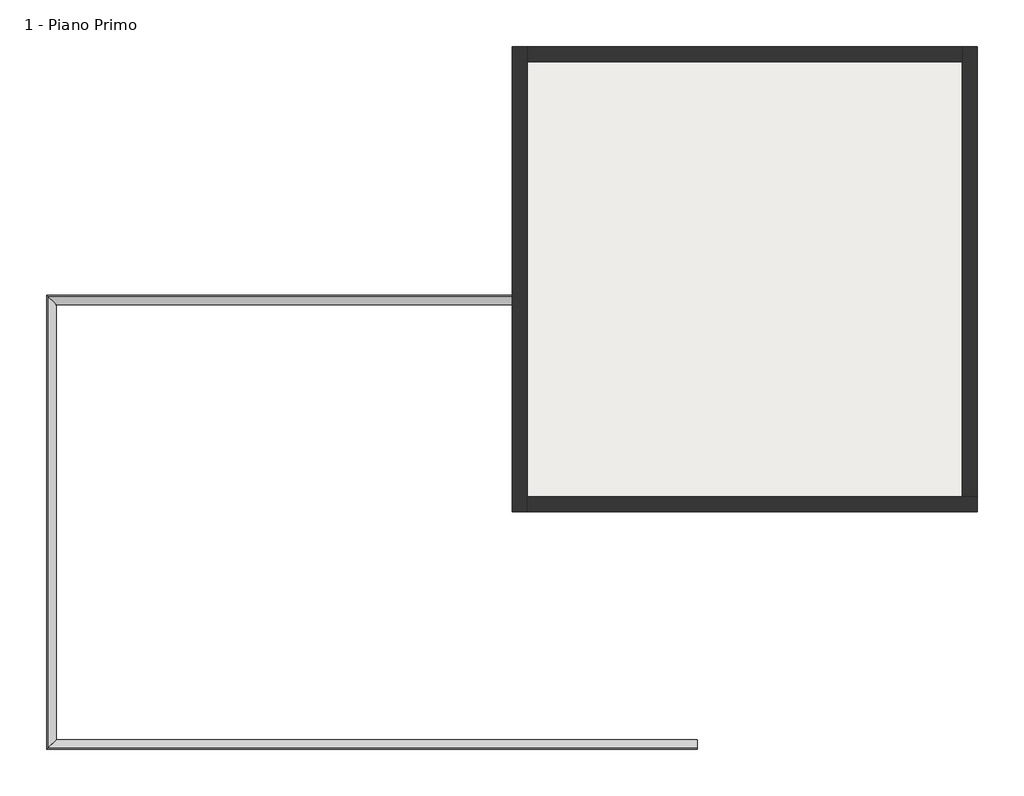
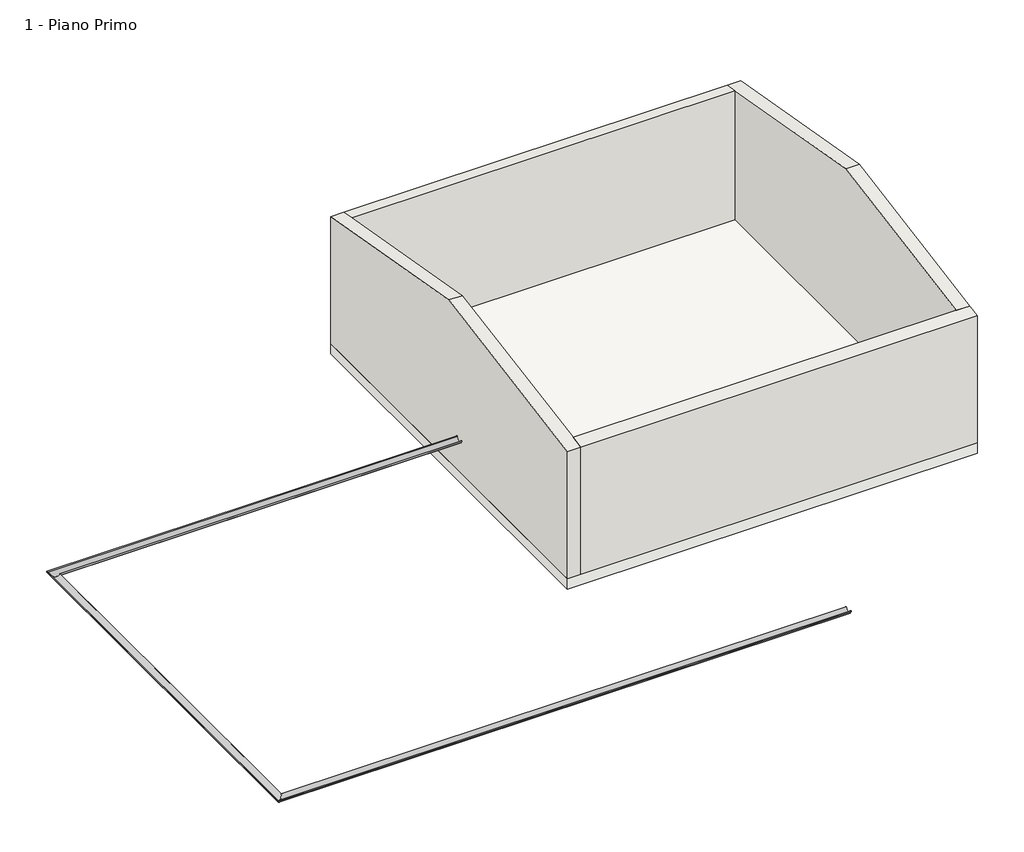
# One storey: 4 walls, 1 pipe segment, 1 slab.
"""IFC4 building model written with IfcOpenShell, lengths in millimetres."""

import ifcopenshell
import ifcopenshell.guid

model = None  # the IFC model being written
_history = None  # IfcOwnerHistory: only IFC2X3 demands one
_inside = {}  # id of a spatial element -> (the spatial element, [elements in it])
_under = {}  # id of a project, library or spatial element -> (it, [spatial elements below it])
_declared = {}  # id of a project -> (the project, [libraries it declares])
_typed = {}  # id of a type object -> (the type object, [elements of that type])
_made_of = {}  # id of a material, layer set ... -> (it, [elements and type objects made of it])


def new_model(schema):
    """Start an empty IFC model of exactly this schema.

    Asked for "IFC4X3", IfcOpenShell would pick the latest addendum, in which some entities
    have other attributes; the version numbers below select the first issue.
    IFC2X3 requires an IfcOwnerHistory on every rooted entity: one is made here for all.
    """
    global model, _history
    if schema == "IFC4X3":
        model = ifcopenshell.file(schema_version=(4, 3, 0, 0))
    else:
        model = ifcopenshell.file(schema=schema)
    _inside.clear()
    _under.clear()
    _declared.clear()
    _typed.clear()
    _made_of.clear()
    _history = None
    if model.schema == "IFC2X3":
        org = make("IfcOrganization", Name="unknown")
        user = make(
            "IfcPersonAndOrganization",
            ThePerson=make("IfcPerson", FamilyName="unknown"),
            TheOrganization=org,
        )
        app = make(
            "IfcApplication",
            ApplicationDeveloper=org,
            Version="unknown",
            ApplicationFullName="unknown",
            ApplicationIdentifier="unknown",
        )
        _history = make(
            "IfcOwnerHistory",
            OwningUser=user,
            OwningApplication=app,
            ChangeAction="ADDED",
            CreationDate=0,
        )
    return model


def make(cls, **values):
    """One entity of the class cls with the attributes given. An attribute that is None is left unset."""
    return model.create_entity(
        cls, **{name: value for name, value in values.items() if value is not None}
    )


def rooted(cls, **values):
    """An entity with a GlobalId (a new one), such as an element, a storey or a relation."""
    return make(cls, GlobalId=ifcopenshell.guid.new(), OwnerHistory=_history, **values)


def si_unit(unit_type, name, prefix=None):
    """IfcSIUnit, for example si_unit("LENGTHUNIT", "METRE", prefix="MILLI")."""
    return make("IfcSIUnit", UnitType=unit_type, Prefix=prefix, Name=name)


def assignment(units):
    """IfcUnitAssignment: the units of a project."""
    return None if units is None else make("IfcUnitAssignment", Units=units)


def point(xyz):
    """IfcCartesianPoint."""
    return None if xyz is None else make("IfcCartesianPoint", Coordinates=xyz)


def direction(xyz):
    """IfcDirection."""
    return None if xyz is None else make("IfcDirection", DirectionRatios=xyz)


def frame(location, z_axis=None, x_axis=None):
    """IfcAxis2Placement3D, a coordinate frame: its origin and axes. An axis left out is left unset."""
    return make(
        "IfcAxis2Placement3D",
        Location=point(location),
        Axis=direction(z_axis),
        RefDirection=direction(x_axis),
    )


def origin():
    """The frame at (0, 0, 0) with its axes left unset."""
    return frame((0.0, 0.0, 0.0))


def place(relative_to, where):
    """IfcLocalPlacement: puts the frame where relative to a parent placement (None: the world)."""
    return make(
        "IfcLocalPlacement", PlacementRelTo=relative_to, RelativePlacement=where
    )


def context(
    kind, dimensions, precision=None, world=None, true_north=None, identifier=None
):
    """IfcGeometricRepresentationContext, for example the 3D "Model" context."""
    return make(
        "IfcGeometricRepresentationContext",
        ContextIdentifier=identifier,
        ContextType=kind,
        CoordinateSpaceDimension=dimensions,
        Precision=precision,
        WorldCoordinateSystem=world,
        TrueNorth=true_north,
    )


def project(units=None, contexts=None):
    """IfcProject with its units and contexts."""
    return rooted(
        "IfcProject",
        Name="project",
        RepresentationContexts=contexts,
        UnitsInContext=assignment(units),
    )


def spatial(cls, under=None, at=None, **own):
    """A site, building, storey or space (cls), placed at a placement, below another one or the project."""
    s = rooted(cls, ObjectPlacement=at, **own)
    if under is not None:
        _under.setdefault(under.id(), (under, []))[1].append(s)
    return s


def polyline(points):
    """IfcPolyline through the points."""
    return make("IfcPolyline", Points=[point(p) for p in points])


def circle_curve(where, radius):
    """IfcCircle in the frame where."""
    return make("IfcCircle", Position=where, Radius=radius)


def ellipse_curve(where, semi_axis1, semi_axis2):
    """IfcEllipse in the frame where."""
    return make(
        "IfcEllipse", Position=where, SemiAxis1=semi_axis1, SemiAxis2=semi_axis2
    )


def outline(outer, holes=None, kind="AREA"):
    """IfcArbitraryClosedProfileDef: a profile drawn as a closed curve; with holes, ...WithVoids."""
    if holes is None:
        return make("IfcArbitraryClosedProfileDef", ProfileType=kind, OuterCurve=outer)
    return make(
        "IfcArbitraryProfileDefWithVoids",
        ProfileType=kind,
        OuterCurve=outer,
        InnerCurves=holes,
    )


def extrude(swept, where, along, depth):
    """IfcExtrudedAreaSolid: the profile swept, set in the frame where, extruded along a direction by depth."""
    return make(
        "IfcExtrudedAreaSolid",
        SweptArea=swept,
        Position=where,
        ExtrudedDirection=direction(along),
        Depth=depth,
    )


def faces_of(points, faces, orient=None, outer=None):
    """IfcFace entities. A face is a list of loops; a loop is a list of indices into points, from 0.

    orient and outer hold one flag for each loop. By default every Orientation is true, the
    first loop of a face is its IfcFaceOuterBound and the others are IfcFaceBound.
    """
    made = []
    for i, loops in enumerate(faces):
        bounds = []
        for j, loop in enumerate(loops):
            is_outer = j == 0 if outer is None else outer[i][j]
            bounds.append(
                make(
                    "IfcFaceOuterBound" if is_outer else "IfcFaceBound",
                    Bound=make("IfcPolyLoop", Polygon=[points[k] for k in loop]),
                    Orientation=True if orient is None else orient[i][j],
                )
            )
        made.append(make("IfcFace", Bounds=bounds))
    return made


def faceted_brep(points, faces, orient=None, outer=None, voids=None):
    """IfcFacetedBrep: a solid bounded by flat faces; with voids (closed shells), ...WithVoids."""
    shared = [point(p) for p in points]
    hull = make("IfcClosedShell", CfsFaces=faces_of(shared, faces, orient, outer))
    if voids is None:
        return make("IfcFacetedBrep", Outer=hull)
    return make(
        "IfcFacetedBrepWithVoids",
        Outer=hull,
        Voids=[
            make(cls, CfsFaces=faces_of(shared, fs, o, b)) for cls, fs, o, b in voids
        ],
    )


def shape(context_of_items, identifier, shape_type, items):
    """IfcShapeRepresentation: the items that make up one representation, for example the "Body"."""
    return make(
        "IfcShapeRepresentation",
        ContextOfItems=context_of_items,
        RepresentationIdentifier=identifier,
        RepresentationType=shape_type,
        Items=items,
    )


def made_of(thing, what):
    """Note that an element or type object is made of a material, layer set ...; save() writes the relation."""
    if what is not None:
        _made_of.setdefault(what.id(), (what, []))[1].append(thing)
    return thing


def element(
    cls,
    number,
    at=None,
    inside=None,
    cuts=None,
    type_object=None,
    material=None,
    context=None,
    identifier="Body",
    shape_type=None,
    held_by="IfcProductDefinitionShape",
    body=None,
    shapes=None,
    **own,
):
    """One element of the class cls, such as IfcWall. Its Tag is "e" and its number.

    at: its placement. inside: the storey or other place that contains it. cuts: it is an
    opening in that element (IfcRelVoidsElement). A single representation is given by context,
    identifier, shape_type and body (its items); several are given by shapes. held_by: the class
    of the entity that holds the representations. save() writes the other relations.
    """
    e = rooted(cls, Tag="e%d" % number, ObjectPlacement=at, **own)
    if body is not None:
        shapes = [shape(context, identifier, shape_type, body)]
    if shapes is not None:
        e.Representation = make(held_by, Representations=shapes)
    if inside is not None:
        _inside.setdefault(inside.id(), (inside, []))[1].append(e)
    if cuts is not None:
        rooted(
            "IfcRelVoidsElement", RelatingBuildingElement=cuts, RelatedOpeningElement=e
        )
    if type_object is not None:
        _typed.setdefault(type_object.id(), (type_object, []))[1].append(e)
    return made_of(e, material)


def aggregate(whole, parts):
    """IfcRelAggregates: a whole, such as a stair, and the parts it consists of."""
    return rooted("IfcRelAggregates", RelatingObject=whole, RelatedObjects=parts)


def save(model, path):
    """Write the relations noted so far, then the file.

    IfcRelAggregates (storeys below a building ...), IfcRelContainedInSpatialStructure (elements
    in a storey), IfcRelDefinesByType, IfcRelAssociatesMaterial and IfcRelDeclares: one each for
    every whole, place, type object, material and project.
    """
    for whole, parts in _under.values():
        aggregate(whole, parts)
    for where, things in _inside.values():
        rooted(
            "IfcRelContainedInSpatialStructure",
            RelatedElements=things,
            RelatingStructure=where,
        )
    for kind, things in _typed.values():
        rooted("IfcRelDefinesByType", RelatedObjects=things, RelatingType=kind)
    for what, things in _made_of.values():
        rooted("IfcRelAssociatesMaterial", RelatedObjects=things, RelatingMaterial=what)
    for by, libraries in _declared.values():
        rooted("IfcRelDeclares", RelatingContext=by, RelatedDefinitions=libraries)
    model.write(path)


def plane_surface(at):
    """IfcPlane: the flat surface through the origin of the frame at, square to its z axis."""
    return make("IfcPlane", Position=at)


def cylinder_surface(at, radius):
    """IfcCylindricalSurface: all points at the distance radius from the z axis of the frame at."""
    return make("IfcCylindricalSurface", Position=at, Radius=radius)


def revolved_surface(curve, axis_point, axis_direction):
    """IfcSurfaceOfRevolution: the curve turned about the line through axis_point along axis_direction."""
    return make(
        "IfcSurfaceOfRevolution",
        SweptCurve=make("IfcArbitraryOpenProfileDef", ProfileType="CURVE", Curve=curve),
        AxisPosition=make("IfcAxis1Placement", Location=point(axis_point), Axis=direction(axis_direction)),
    )


def advanced_brep(points, edges, surfaces, faces):
    """IfcAdvancedBrep: a solid bounded by faces that lie on surfaces and meet in shared edges.

    An edge is (start, end): straight between two places in points (the first is 0);
    or (start, end, curve); or (start, end, curve, False) where it runs against its curve.
    A face is (place in surfaces, loops), or (place, loops, False) where it looks against
    its surface's normal. A loop lists edges by number (the first is 1), with a minus sign
    where the edge is run from its end to its start. The first loop is the outer one.
    """
    corners = [point(p) for p in points]
    vertices = [make("IfcVertexPoint", VertexGeometry=c) for c in corners]
    made = []
    for start, end, *more in edges:
        made.append(
            make(
                "IfcEdgeCurve",
                EdgeStart=vertices[start],
                EdgeEnd=vertices[end],
                EdgeGeometry=more[0] if more else make("IfcPolyline", Points=[corners[start], corners[end]]),
                SameSense=more[1] if len(more) > 1 else True,
            )
        )
    hull = []
    for where, loops, *sense in faces:
        bounds = []
        for j, loop in enumerate(loops):
            ring = [make("IfcOrientedEdge", EdgeElement=made[abs(k) - 1], Orientation=k > 0) for k in loop]
            bounds.append(
                make(
                    "IfcFaceOuterBound" if j == 0 else "IfcFaceBound",
                    Bound=make("IfcEdgeLoop", EdgeList=ring),
                    Orientation=True,
                )
            )
        hull.append(make("IfcAdvancedFace", Bounds=bounds, FaceSurface=surfaces[where], SameSense=sense[0] if sense else True))
    return make("IfcAdvancedBrep", Outer=make("IfcClosedShell", CfsFaces=hull))


model = new_model("IFC4")

# Units and contexts
model_context = context("Model", 3, world=origin())
ifc_project = project(units=[si_unit("LENGTHUNIT", "METRE", prefix="MILLI")], contexts=[model_context])

# Site, building, storey
site = spatial("IfcSite", under=ifc_project)
building = spatial("IfcBuilding", under=site)
storey = spatial("IfcBuildingStorey", under=building, Name="1 - Piano Primo", Elevation=4000.0)

# Pipe segment
placement = place(None, origin())
element("IfcPipeSegment", 1, ObjectType="Grondaia", at=placement, inside=storey, context=model_context, shape_type="AdvancedBrep", body=[
    advanced_brep(
    [(-1450.292668, 3378.2301644, 4973.2050808), (-1450.292668, 3588.4212472, 4973.2050808), (-1450.292668, 3586.4212472, 4973.2050808), (-1450.292668, 3380.2301644, 4973.2050808), (-1450.292668, 3368.2301644, 4961.2050808), (-1450.292668, 3368.2301644, 4963.2050808), (-17240.4837508, 3368.2301644, 4963.2050808), (-17230.4837508, 3378.2301644, 4973.2050808), (-17240.4837508, 3368.2301644, 4961.2050808), (-17228.4837508, 3380.2301644, 4973.2050808), (-17022.292668, 3586.4212472, 4973.2050808), (-17020.292668, 3588.4212472, 4973.2050808), (-17240.4837508, 14378.61233, 4963.2050808), (-17230.4837508, 14368.61233, 4973.2050808), (-17240.4837508, 14378.61233, 4961.2050808), (-17228.4837508, 14366.61233, 4973.2050808), (-17022.292668, 14160.4212472, 4973.2050808), (-17020.292668, 14158.4212472, 4973.2050808), (-5941.300812, 14368.61233, 4973.2050808), (-5941.300812, 14378.61233, 4963.2050808), (-5941.300812, 14378.61233, 4961.2050808), (-5941.300812, 14366.61233, 4973.2050808), (-5941.300812, 14160.4212472, 4973.2050808), (-5941.300812, 14158.4212472, 4973.2050808)],
    [
        (0, 1, circle_curve(frame((-1450.292668, 3483.3257058, 4973.2050808), z_axis=(1.0, 0.0, 0.0), x_axis=(0.0, -1.0, 0.0)), 105.0955414)),
        (1, 2),
        (2, 3, circle_curve(frame((-1450.292668, 3483.3257058, 4973.2050808), z_axis=(-1.0, 0.0, 0.0), x_axis=(0.0, -1.0, 0.0)), 103.0955414)),
        (3, 4, circle_curve(frame((-1450.292668, 3368.2301644, 4973.2050808), z_axis=(1.0, 0.0, 0.0), x_axis=(0.0, -1.0, 0.0)), 12.0)),
        (4, 5),
        (5, 0, circle_curve(frame((-1450.292668, 3368.2301644, 4973.2050808), z_axis=(-1.0, 0.0, 0.0), x_axis=(0.0, -1.0, 0.0)), 10.0)),
        (6, 7, ellipse_curve(frame((-17240.4837508, 3368.2301644, 4973.2050808), z_axis=(-0.7071067811865469, 0.7071067811865481, 0.0), x_axis=(0.7071067811865481, 0.7071067811865468, 0.0)), 14.1421356, 10.0)),
        (7, 0),
        (5, 6),
        (8, 6),
        (4, 8),
        (9, 8, ellipse_curve(frame((-17240.4837508, 3368.2301644, 4973.2050808), z_axis=(0.7071067811865469, -0.7071067811865481, 0.0), x_axis=(-0.7071067811865481, -0.7071067811865468, 0.0)), 16.9705627, 12.0)),
        (3, 9),
        (10, 9, ellipse_curve(frame((-17125.3882094, 3483.3257058, 4973.2050808), z_axis=(-0.7071067811865469, 0.7071067811865481, 0.0), x_axis=(0.7071067811865481, 0.7071067811865468, 0.0)), 145.7991129, 103.0955414)),
        (2, 10),
        (11, 10),
        (1, 11),
        (7, 11, ellipse_curve(frame((-17125.3882094, 3483.3257058, 4973.2050808), z_axis=(0.7071067811865469, -0.7071067811865481, 0.0), x_axis=(-0.7071067811865481, -0.7071067811865468, 0.0)), 148.62754, 105.0955414)),
        (12, 13, ellipse_curve(frame((-17240.4837508, 14378.61233, 4973.2050808), z_axis=(0.7071067811865491, 0.7071067811865458, 0.0), x_axis=(0.7071067811865456, -0.7071067811865493, 0.0)), 14.1421356, 10.0)),
        (13, 7),
        (6, 12),
        (14, 12),
        (8, 14),
        (15, 14, ellipse_curve(frame((-17240.4837508, 14378.61233, 4973.2050808), z_axis=(-0.7071067811865491, -0.7071067811865458, 0.0), x_axis=(-0.7071067811865456, 0.7071067811865493, 0.0)), 16.9705627, 12.0)),
        (9, 15),
        (16, 15, ellipse_curve(frame((-17125.3882094, 14263.5167886, 4973.2050808), z_axis=(0.7071067811865491, 0.7071067811865458, 0.0), x_axis=(0.7071067811865456, -0.7071067811865493, 0.0)), 145.7991129, 103.0955414)),
        (10, 16),
        (17, 16),
        (11, 17),
        (13, 17, ellipse_curve(frame((-17125.3882094, 14263.5167886, 4973.2050808), z_axis=(-0.7071067811865491, -0.7071067811865458, 0.0), x_axis=(-0.7071067811865456, 0.7071067811865493, 0.0)), 148.62754, 105.0955414)),
        (18, 19, circle_curve(frame((-5941.300812, 14378.61233, 4973.2050808), z_axis=(-1.0, 0.0, 0.0), x_axis=(0.0, 1.0, 0.0)), 10.0)),
        (19, 20),
        (20, 21, circle_curve(frame((-5941.300812, 14378.61233, 4973.2050808), z_axis=(1.0, 0.0, 0.0), x_axis=(0.0, 1.0, 0.0)), 12.0)),
        (21, 22, circle_curve(frame((-5941.300812, 14263.5167886, 4973.2050808), z_axis=(-1.0, 0.0, 0.0), x_axis=(0.0, 1.0, 0.0)), 103.0955414)),
        (22, 23),
        (23, 18, circle_curve(frame((-5941.300812, 14263.5167886, 4973.2050808), z_axis=(1.0, 0.0, 0.0), x_axis=(0.0, 1.0, 0.0)), 105.0955414)),
        (18, 13),
        (12, 19),
        (14, 20),
        (15, 21),
        (16, 22),
        (17, 23),
    ],
    [
        plane_surface(frame((-1450.292668, 3588.4212472, 4741.5716357), z_axis=(1.0, 0.0, 0.0), x_axis=(0.0, 1.0, 0.0))),
        revolved_surface(polyline([(-1450.292668, 3358.2301644, 4973.2050808), (-17250.483750783216, 3358.2301644, 4973.2050808)]), (-17020.292668, 3368.2301644, 4973.2050808), (1.0, 0.0, 0.0)),
        plane_surface(frame((-17240.4837508, 3368.2301644, 4963.2050808), z_axis=(0.0, 1.0, 0.0), x_axis=(1.0, 0.0, 0.0))),
        cylinder_surface(frame((-17020.292668, 3368.2301644, 4973.2050808), z_axis=(-1.0, 0.0, 0.0), x_axis=(0.0, -1.0, 0.0)), 12.0),
        revolved_surface(polyline([(-1450.292668, 3380.2301644, 4973.2050808), (-17228.483750822572, 3380.2301644, 4973.2050808)]), (-17020.292668, 3483.3257058, 4973.2050808), (1.0, 0.0, 0.0)),
        plane_surface(frame((-17022.292668, 3586.4212472, 4973.2050808), z_axis=(0.0, 0.0, 1.0), x_axis=(1.0, 0.0, 0.0))),
        cylinder_surface(frame((-17020.292668, 3483.3257058, 4973.2050808), z_axis=(-1.0, 0.0, 0.0), x_axis=(0.0, -1.0, 0.0)), 105.0955414),
        revolved_surface(polyline([(-17250.4837508, 3358.23016441678, 4973.2050808), (-17250.4837508, 14388.61232998322, 4973.2050808)]), (-17240.4837508, 14158.4212472, 4973.2050808), (0.0, -1.0, 0.0)),
        plane_surface(frame((-17240.4837508, 14378.61233, 4963.2050808), z_axis=(1.0, 0.0, 0.0), x_axis=(0.0, -1.0, 0.0))),
        cylinder_surface(frame((-17240.4837508, 14158.4212472, 4973.2050808), z_axis=(0.0, 1.0, 0.0), x_axis=(-1.0, 0.0, 0.0)), 12.0),
        revolved_surface(polyline([(-17228.4837508, 3380.2301643774263, 4973.2050808), (-17228.4837508, 14366.612330022574, 4973.2050808)]), (-17125.3882094, 14158.4212472, 4973.2050808), (0.0, -1.0, 0.0)),
        plane_surface(frame((-17022.292668, 14160.4212472, 4973.2050808), z_axis=(0.0, 0.0, 1.0), x_axis=(0.0, -1.0, 0.0))),
        cylinder_surface(frame((-17125.3882094, 14158.4212472, 4973.2050808), z_axis=(0.0, 1.0, 0.0), x_axis=(-1.0, 0.0, 0.0)), 105.0955414),
        plane_surface(frame((-5941.300812, 14158.4212472, 4741.5716357), z_axis=(1.0, 0.0, 0.0), x_axis=(0.0, -1.0, 0.0))),
        revolved_surface(polyline([(-17250.483750783216, 14388.61233, 4973.2050808), (-5941.300812, 14388.61233, 4973.2050808)]), (-5941.300812, 14378.61233, 4973.2050808), (-1.0, 0.0, 0.0)),
        plane_surface(frame((-5941.300812, 14378.61233, 4963.2050808), z_axis=(0.0, -1.0, 0.0), x_axis=(-1.0, 0.0, 0.0))),
        cylinder_surface(frame((-5941.300812, 14378.61233, 4973.2050808), z_axis=(1.0, 0.0, 0.0), x_axis=(0.0, 1.0, 0.0)), 12.0),
        revolved_surface(polyline([(-17228.483750822572, 14366.61233, 4973.2050808), (-5941.300812, 14366.61233, 4973.2050808)]), (-5941.300812, 14263.5167886, 4973.2050808), (-1.0, 0.0, 0.0)),
        plane_surface(frame((-5941.300812, 14160.4212472, 4973.2050808), z_axis=(0.0, 0.0, 1.0), x_axis=(-1.0, 0.0, 0.0))),
        cylinder_surface(frame((-5941.300812, 14263.5167886, 4973.2050808), z_axis=(1.0, 0.0, 0.0), x_axis=(0.0, 1.0, 0.0)), 105.0955414),
    ],
    [
        (0, [[1, 2, 3, 4, 5, 6]]),
        (1, [[7, 8, -6, 9]]),
        (2, [[10, -9, -5, 11]]),
        (3, [[12, -11, -4, 13]]),
        (4, [[14, -13, -3, 15]]),
        (5, [[16, -15, -2, 17]]),
        (6, [[18, -17, -1, -8]]),
        (7, [[19, 20, -7, 21]]),
        (8, [[22, -21, -10, 23]]),
        (9, [[24, -23, -12, 25]]),
        (10, [[26, -25, -14, 27]]),
        (11, [[28, -27, -16, 29]]),
        (12, [[30, -29, -18, -20]]),
        (13, [[31, 32, 33, 34, 35, 36]]),
        (14, [[-31, 37, -19, 38]]),
        (15, [[-32, -38, -22, 39]]),
        (16, [[-33, -39, -24, 40]]),
        (17, [[-34, -40, -26, 41]]),
        (18, [[-35, -41, -28, 42]]),
        (19, [[-36, -42, -30, -37]]),
    ],
),
])

# Slab
element("IfcSlab", 2, ObjectType="Latero Cementizio - 30 cm", at=placement, inside=storey, context=model_context, shape_type="SweptSolid", body=[
    extrude(outline(polyline([(-5941.300812, 20428.4386987), (5358.699188, 20428.4386987), (5358.699188, 9128.4386987), (-5941.300812, 9128.4386987), (-5941.300812, 20428.4386987)])), frame((0.0, 0.0, 3700.0), z_axis=(0.0, 0.0, 1.0), x_axis=(1.0, 0.0, 0.0)), (0.0, 0.0, 1.0), 300.0),
])

# Walls
element("IfcWall", 3, ObjectType="37 cm", at=placement, inside=storey, context=model_context, shape_type="Brep", body=[
    faceted_brep([(-5941.300812, 20428.4386987, 4000.0), (-5941.300812, 9128.4386987, 4000.0), (-5941.300812, 9128.4386987, 7700.0), (-5941.300812, 14778.4386987, 8696.247441), (-5941.300812, 20428.4386987, 7700.0), (-5571.300812, 20428.4386987, 4000.0), (-5571.300812, 20428.4386987, 7700.0), (-5571.300812, 20058.4386987, 7765.2409829), (-5571.300812, 14778.4386987, 8696.247441), (-5571.300812, 9498.4386987, 7765.2409829), (-5571.300812, 9128.4386987, 7700.0), (-5571.300812, 9128.4386987, 4000.0), (-5571.300812, 9498.4386987, 4000.0), (-5571.300812, 20058.4386987, 4000.0)], [[[0, 1, 2, 3, 4]], [[5, 6, 7, 8, 9, 10, 11, 12, 13]], [[1, 0, 5, 13, 12, 11]], [[2, 1, 11, 10]], [[0, 4, 6, 5]], [[4, 3, 8, 7, 6]], [[3, 2, 10, 9, 8]]]),
])
element("IfcWall", 4, ObjectType="37 cm", at=placement, inside=storey, context=model_context, shape_type="Brep", body=[
    faceted_brep([(-5571.300812, 9128.4386987, 4000.0), (5358.699188, 9128.4386987, 4000.0), (5358.699188, 9128.4386987, 7700.0), (-5571.300812, 9128.4386987, 7700.0), (-5571.300812, 9498.4386987, 4000.0), (-5571.300812, 9498.4386987, 7765.2409829), (4988.699188, 9498.4386987, 7765.2409829), (5358.699188, 9498.4386987, 7765.2409829), (5358.699188, 9498.4386987, 4000.0), (4988.699188, 9498.4386987, 4000.0)], [[[0, 1, 2, 3]], [[4, 5, 6, 7, 8, 9]], [[1, 0, 4, 9, 8]], [[0, 3, 5, 4]], [[2, 1, 8, 7]], [[3, 2, 7, 6, 5]]]),
])
element("IfcWall", 5, ObjectType="37 cm", at=placement, inside=storey, context=model_context, shape_type="Brep", body=[
    faceted_brep([(5358.699188, 9498.4386987, 4000.0), (5358.699188, 20428.4386987, 4000.0), (5358.699188, 20428.4386987, 7700.0), (5358.699188, 14778.4386987, 8696.247441), (5358.699188, 9498.4386987, 7765.2409829), (4988.699188, 9498.4386987, 4000.0), (4988.699188, 9498.4386987, 7765.2409829), (4988.699188, 14778.4386987, 8696.247441), (4988.699188, 20058.4386987, 7765.2409829), (4988.699188, 20428.4386987, 7700.0), (4988.699188, 20428.4386987, 4000.0), (4988.699188, 20058.4386987, 4000.0)], [[[0, 1, 2, 3, 4]], [[5, 6, 7, 8, 9, 10, 11]], [[1, 0, 5, 11, 10]], [[0, 4, 6, 5]], [[2, 1, 10, 9]], [[4, 3, 7, 6]], [[3, 2, 9, 8, 7]]]),
])
element("IfcWall", 6, ObjectType="37 cm", at=placement, inside=storey, context=model_context, shape_type="SweptSolid", body=[
    extrude(outline(polyline([(20428.4386987, 7700.0), (20428.4386987, 4000.0), (20058.4386987, 4000.0), (20058.4386987, 7765.2409829), (20428.4386987, 7700.0)])), frame((-5571.300812, 0.0, 0.0), z_axis=(1.0, 0.0, 0.0), x_axis=(0.0, 1.0, 0.0)), (0.0, 0.0, 1.0), 10560.0),
])

save(model, "model.ifc")

# Revit data of these elements
# Type "Latero Cementizio - 30 cm"
#   Keynote = "S/3"
#   Function = 0
#   Layers, outside or top first: 0.02 m "Ceramica bianca" (function 4); 0.065 m "Sabbia e Calcestruzzo" (function 2); 0.04 m "Calcestruzzo" (function 1); 0.16 m "Laterizio (2)" (function 1); 0.015 m "Intonaco - Bianco" (function 5)
# Type "37 cm"
#   Keynote = "Mb/3"
#   Layers, outside or top first: 0.02 m "Intonaco esterno" (function 1); 0.08 m "Isolamento" (function 1); 0.25 m "Calcestruzzo Blocchi" (function 1); 0.02 m "Intonaco interno" (function 5)
# Element 1 (IfcPipeSegment, "Grondaia")
#   Phase Created = Stato di Progetto
#   Materials on its faces: "Default - Grondaia"
# Element 2 (IfcSlab, "Latero Cementizio - 30 cm")
#   Height Offset From Level = 0.00 m
#   Phase Created = Stato di Progetto
#   Materials on its faces: "Intonaco - Bianco", "Ceramica bianca"
# Element 3 (IfcWall, "37 cm")
#   Top Offset = 0.00 m
#   Base Offset = 0.00 m
#   Unconnected Height = 3.70 m
#   wall height = 3.70 m
#   Phase Created = Stato di Progetto
#   Base Constraint = 1 - Piano Primo
#   Materials on its faces: "Intonaco interno", "Default - Calcestruzzo", "Intonaco esterno"
# Elements 4, 5, 6 (IfcWall, "37 cm")
#   Top Offset = 0.00 m
#   Base Offset = 0.00 m
#   Unconnected Height = 3.70 m
#   wall height = 3.70 m
#   Phase Created = Stato di Progetto
#   Base Constraint = 1 - Piano Primo
#   Materials on its faces: "Default - Calcestruzzo", "Intonaco interno", "Intonaco esterno"
# Materials
#   "Ceramica bianca": class "Ceramica", colour RGB 210 210 210, transparency 0, Description = "Finitura interna - Piastrelle di ceramica incollate", Cost = 0
#   "Sabbia e Calcestruzzo": class "Calcestruzzo", colour RGB 127 127 127, transparency 0, Description = "Magrone - Sabbia e cemento", Cost = 0
#   "Calcestruzzo": class "Calcestruzzo", colour RGB 192 192 192, transparency 0, Description = "Calcestruzzo - Cemento Portland", Cost = 0
#   "Laterizio (2)": class "Mattone", colour RGB 255 128 64, transparency 0, Description = "Pignatta h 16 cm", Cost = 0
#   "Intonaco - Bianco": class "Intonaco", colour RGB 249 249 249, transparency 0, Description = "Verniciatura", Cost = 0
#   "Intonaco esterno": class "Intonaco", colour RGB 249 249 249, transparency 0, Description = "Verniciatura", Cost = 0
#   "Isolamento": class "Varie", colour RGB 127 127 127, transparency 0, Description = "Pannello in sughero", Cost = 0
#   "Calcestruzzo Blocchi": class "Calcestruzzo", colour RGB 255 128 0, transparency 0, Description = "Calcestruzzo - Cemento Portland", Cost = 0
#   "Intonaco interno": class "Intonaco", colour RGB 249 249 249, transparency 0, Description = "Verniciatura", Cost = 0
#   "Default - Grondaia": class "Varie", colour RGB 212 140 110, transparency 0, Description = "Legno di pino", Cost = 0
#   "Default - Calcestruzzo": class "Calcestruzzo", colour RGB 192 192 192, transparency 0, Description = "Calcestruzzo", Cost = 0
